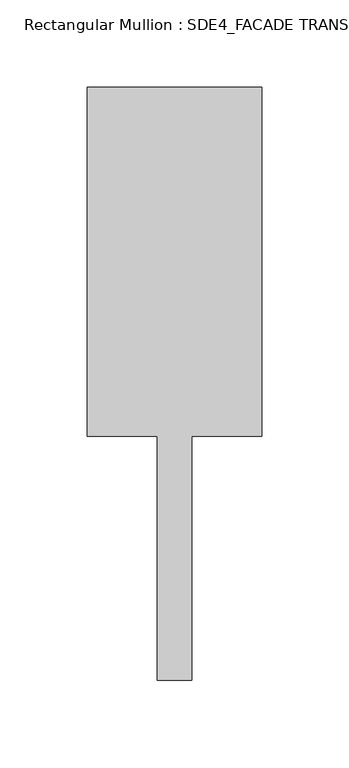
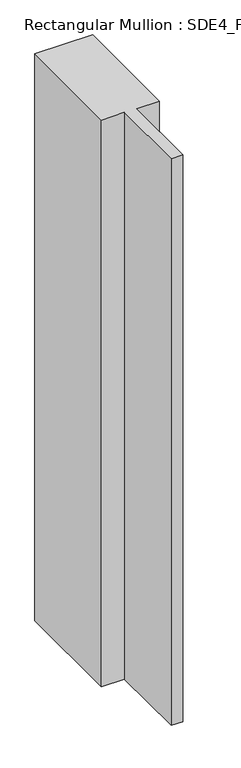
"""IFC4 building model written with IfcOpenShell, lengths in millimetres: member geometry, Rectangular Mullion : SDE4_FACADE TRANSOM TYPE 1."""

from ifc_helpers import new_model, si_unit, frame, origin, place, context, project, spatial, polyline, outline, extrude, source, transform, mapped, element, save


def rectangular_mullion_sde4_facade_transom_type_1_2c6e8619(model_context):
    return source(origin(), model_context, "Body", "SweptSolid", [
        extrude(outline(polyline([(50.0, 132.5), (50.0, -67.5), (10.0, -67.5), (10.0, -207.5), (-10.0, -207.5), (-10.0, -67.5), (-50.0, -67.5), (-50.0, 132.5), (50.0, 132.5)])), frame((0.0, 0.0, -1040.0), z_axis=(0.0, 0.0, 1.0), x_axis=(1.0, 0.0, 0.0)), (0.0, 0.0, 1.0), 1040.0),
    ])


if __name__ == "__main__":
    model = new_model("IFC4")
    model_context = context("Model", 3, world=origin())
    ifc_project = project(units=[si_unit("LENGTHUNIT", "METRE", prefix="MILLI")], contexts=[model_context])
    site = spatial("IfcSite", under=ifc_project)
    building = spatial("IfcBuilding", under=site)
    placement = place(None, origin())
    rectangular_mullion_sde4_facade_transom_type_1_shape = rectangular_mullion_sde4_facade_transom_type_1_2c6e8619(model_context)
    element("IfcMember", 1, ObjectType="Rectangular Mullion : SDE4_FACADE TRANSOM TYPE 1", at=placement, inside=building, context=model_context, shape_type="MappedRepresentation", body=[
        mapped(rectangular_mullion_sde4_facade_transom_type_1_shape, transform((0.0, 0.0, 0.0), x_axis=(1.0, 0.0, 0.0), y_axis=(0.0, 1.0, 0.0), z_axis=(0.0, 0.0, 1.0))),
    ])
    save(model, "model.ifc")

# Revit data of these elements
# Type "Rectangular Mullion : SDE4_FACADE TRANSOM TYPE 1"
#   built-in parameter 1007322 = 1.11549 (stored number, unit not read)
#   built-in parameter 1007321 = 0.164042 (stored number, unit not read)
#   built-in parameter 1007320 = 0.164042 (stored number, unit not read)
